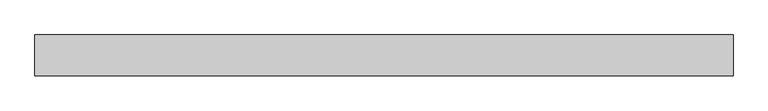
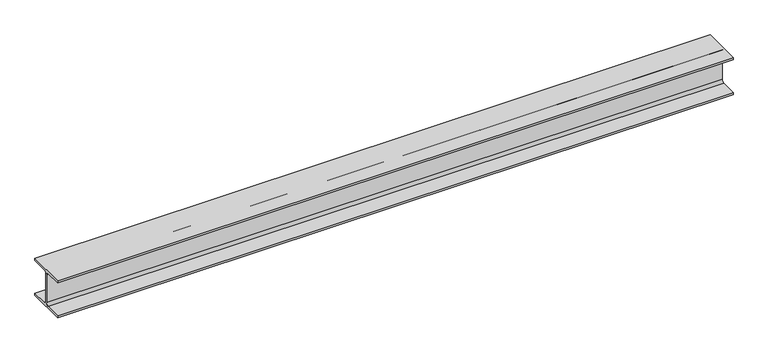
"""IFC4 building model written with IfcOpenShell, lengths in millimetres: beam geometry, 0912_Steel Framing_H-KSD3502 : H_SB_ASB_H-200x200x8x12."""

from ifc_helpers import new_model, si_unit, point, frame, frame_2d, origin, place, context, project, spatial, polyline, circle_curve, trimmed, segment, composite_curve, outline, extrude, source, transform, mapped, element, save


def beam_938f72db(model_context):
    return source(origin(), model_context, "Body", "SweptSolid", [
        extrude(outline(composite_curve([segment(polyline([(100.0, -88.0), (100.0, -100.0), (-100.0, -100.0), (-100.0, -88.0), (-17.0, -88.0)]), True, "CONTINUOUS"), segment(trimmed(circle_curve(frame_2d((-17.0, -75.0)), 13.0), [point((-17.0, -88.0))], [point((-4.0, -75.0))], True, "CARTESIAN"), True, "CONTINUOUS"), segment(polyline([(-4.0, -75.0), (-4.0, 75.0)]), True, "CONTINUOUS"), segment(trimmed(circle_curve(frame_2d((-17.0, 75.0)), 13.0), [point((-4.0, 75.0))], [point((-17.0, 88.0))], True, "CARTESIAN"), True, "CONTINUOUS"), segment(polyline([(-17.0, 88.0), (-100.0, 88.0), (-100.0, 100.0), (100.0, 100.0), (100.0, 88.0), (17.0, 88.0)]), True, "CONTINUOUS"), segment(trimmed(circle_curve(frame_2d((17.0, 75.0)), 13.0), [point((17.0, 88.0))], [point((4.0, 75.0))], True, "CARTESIAN"), True, "CONTINUOUS"), segment(polyline([(4.0, 75.0), (4.0, -75.0)]), True, "CONTINUOUS"), segment(trimmed(circle_curve(frame_2d((17.0, -75.0)), 13.0), [point((4.0, -75.0))], [point((17.0, -88.0))], True, "CARTESIAN"), True, "CONTINUOUS"), segment(polyline([(17.0, -88.0), (100.0, -88.0)]), True, "CONTINUOUS")], self_intersect=False)), frame((-1594.2199273, 0.0, 0.0), z_axis=(1.0, 0.0, 0.0), x_axis=(0.0, 1.0, 0.0)), (0.0, 0.0, 1.0), 3427.8844631),
    ])


if __name__ == "__main__":
    model = new_model("IFC4")
    model_context = context("Model", 3, world=origin())
    ifc_project = project(units=[si_unit("LENGTHUNIT", "METRE", prefix="MILLI")], contexts=[model_context])
    site = spatial("IfcSite", under=ifc_project)
    building = spatial("IfcBuilding", under=site)
    placement = place(None, origin())
    beam_shape = beam_938f72db(model_context)
    element("IfcBeam", 1, ObjectType="0912_Steel Framing_H-KSD3502 : H_SB_ASB_H-200x200x8x12", at=placement, inside=building, context=model_context, shape_type="MappedRepresentation", body=[
        mapped(beam_shape, transform((0.0, 0.0, 0.0), x_axis=(1.0, 0.0, 0.0), y_axis=(0.0, 1.0, 0.0), z_axis=(0.0, 0.0, 1.0))),
    ])
    save(model, "model.ifc")

# Revit data of these elements
# Type "0912_Steel Framing_H-KSD3502 : H_SB_ASB_H-200x200x8x12"
#   H_WM Code_1 = "S01AA002-00001 | Main Steel Structure Fabrication Work | Shelter/Building | Medium Steel - Standard (90KG/M>Weight≥30KG/M) | Material: (   )"
#   H_WM Code_2 = "S03AA028-00001 | Main Steel Structure Erection Work | Shelter/Building | Medium Steel (90KG/M>Weight≥30KG/M) | Material: (   )"
#   H_WM Code_3 = "S01AA010-00001 | Main Steel Structure Fabrication Work | Shelter/Building | Steel Painting/Coating | for Non-Fireproofed Steel Surface, Surface Preparation, Primer, Second & Final Coat | Material: (   )"
#   H_Q'ty Cal Type Tag = "SB-Q2"
#   Width = 20.0 cm
#   Web Thickness = 0.8 cm
#   Web Fillet = 1.3 cm
#   Warping Constant = 141000.0 cm⁶
#   W = 0
#   Torsional Moment of Inertia = 26.2485 cm⁴
#   Section Area = 63.53 cm²
#   Plastic Modulus weak axis = 244.0 cm³
#   Plastic Modulus strong axis = 525.0 cm³
#   Perimeter = 1.16 m²/m
#   Nominal Weight = 49.90 kgf/m
#   Moment of Inertia weak axis = 1600.00 cm⁴
#   Moment of Inertia strong axis = 4720.00 cm⁴
#   Height = 20.0 cm
#   Flange Thickness = 1.2 cm
#   Elastic Modulus weak axis = 160.0 cm³
#   Elastic Modulus strong axis = 472.0 cm³
#   Centroid Vertical = 10.0 cm
#   Centroid Horizontal = 10.0 cm
#   Ix = 47200000
#   Length [instance default] = 1.5240 m
#   Zx = 525000
#   b = 0.2000 m
#   h = 0.2000 m
#   r = 0.0130 m
#   s = 0.0080 m
#   t = 0.0120 m
#   A = 0.006353 m²
#   Structural Material [instance default] = Steel, 45-345
#   Assembly Code = ""
# Element 1 (IfcBeam, "0912_Steel Framing_H-KSD3502 : H_SB_ASB_H-200x200x8x12")
#   Structural Material = none
# Materials
#   "Steel, 45-345": class "Metal", colour RGB 189 187 185, transparency 0, Description = "Steel 345 MPa", Cost = 0
